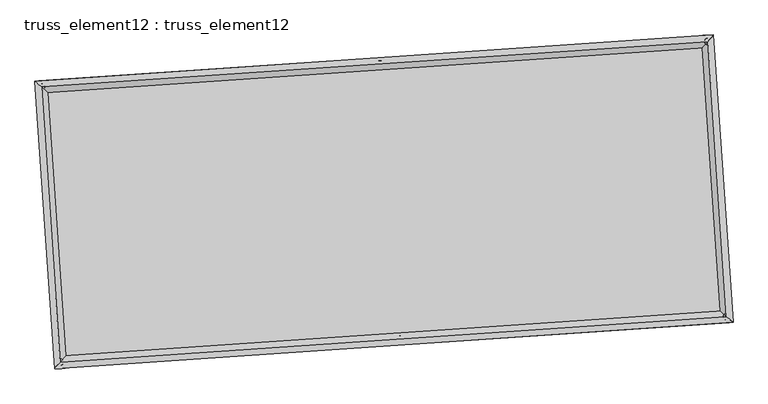
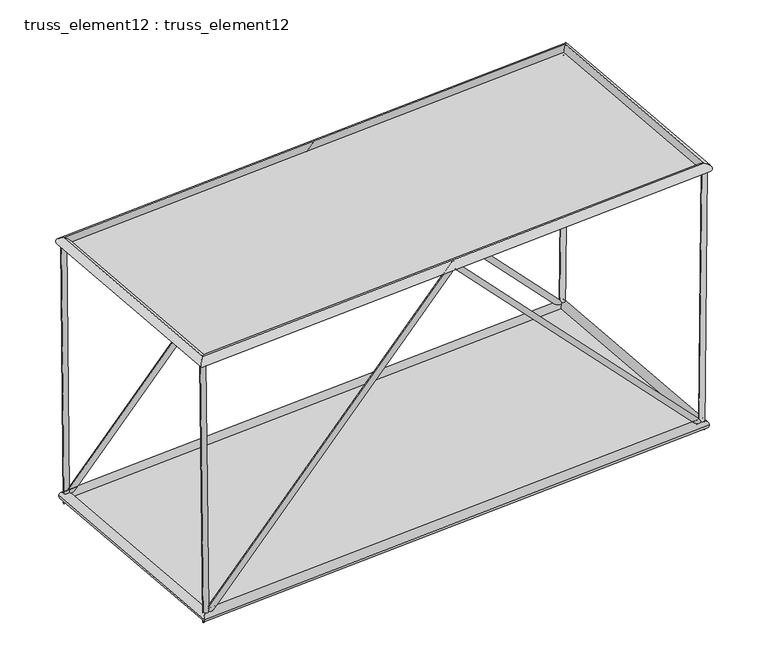
"""IFC4 building model written with IfcOpenShell, lengths in millimetres: plate geometry, truss_element12 : truss_element12."""

from ifc_helpers import new_model, si_unit, frame, origin, origin_with_axes, place, context, project, spatial, polyline, circle_curve, ellipse_curve, outline, extrude, source, transform, mapped, element, save
from ifc_brep_helpers import plane_surface, cylinder_surface, advanced_brep


def truss_element12_truss_element12_25fafcbe(model_context):
    return source(origin(), model_context, "Body", "SolidModel", [
        advanced_brep(
        [(-3717.9336518, 2272.6106472, 5000.2478695), (-3817.0314009, 2259.2497843, 4999.187935), (-3666.2408019, 2276.1353862, 122.8345798), (-3762.7460809, 2262.9512939, -122.8345798), (1064.197845, 2598.6860154, 5071.8345971), (1064.6389029, 2592.1123254, 4927.5910047), (5793.7028088, 2921.1729804, 122.8278987), (5891.0581682, 2921.2075081, -122.8278987), (5846.3222996, 2924.7609034, 5000.2471651), (5946.316249, 2924.9753466, 4999.1682339)],
        [
            (0, 1, circle_curve(frame((-3767.4825264, 2265.9302158, 4999.7179023), z_axis=(-0.01059781698674716, -0.0007226248542523914, 0.9999435804526352), x_axis=(-0.13360875038090175, 0.9910339106331651, -0.0006998548346273042)), 50.0)),
            (1, 0, circle_curve(frame((-3767.4825264, 2265.9302158, 4999.7179023), z_axis=(-0.01059781698674716, -0.0007226248542523914, 0.9999435804526352), x_axis=(-0.13360875038090175, 0.9910339106331651, -0.0006998548346273042)), 50.0)),
            (0, 2),
            (2, 3, ellipse_curve(frame((-3714.4934414, 2269.54334, 0.0), z_axis=(-0.9277371610449594, -0.06325887035254743, 0.36783430418866414), x_axis=(0.36698217779578546, 0.025023119674036753, 0.9298913509986214)), 132.383262, 50.0)),
            (3, 1),
            (3, 2, ellipse_curve(frame((-3714.4934414, 2269.54334, 0.0), z_axis=(-0.9277371610449594, -0.06325887035254743, 0.36783430418866414), x_axis=(0.36698217779578546, 0.025023119674036753, 0.9298913509986214)), 132.383262, 50.0)),
            (2, 4),
            (4, 5, ellipse_curve(frame((1064.418374, 2595.3991704, 4999.7128009), z_axis=(-0.9976833948456157, -0.0680282381448872, 4.9641008010384885e-05), x_axis=(-4.952600945652472e-05, -3.3769903190067476e-06, -0.9999999987678853)), 72.2788404, 50.0)),
            (5, 3),
            (5, 4, ellipse_curve(frame((1064.418374, 2595.3991704, 4999.7128009), z_axis=(-0.9976833948456157, -0.0680282381448872, 4.9641008010384885e-05), x_axis=(-4.952600945652472e-05, -3.3769903190067476e-06, -0.9999999987678853)), 72.2788404, 50.0)),
            (4, 6),
            (6, 7, ellipse_curve(frame((5842.3804885, 2921.1902443, 0.0), z_axis=(-0.9277903039426281, -0.06326249396472418, -0.36769961757854613), x_axis=(-0.3668478032011972, -0.025013957181237265, 0.9299446172931972)), 132.3684791, 50.0)),
            (7, 5),
            (7, 6, ellipse_curve(frame((5842.3804885, 2921.1902443, 0.0), z_axis=(-0.9277903039426281, -0.06326249396472418, -0.36769961757854613), x_axis=(-0.3668478032011972, -0.025013957181237265, 0.9299446172931972)), 132.3684791, 50.0)),
            (8, 9, circle_curve(frame((5896.3192743, 2924.868125, 4999.7076995), z_axis=(0.010787757166797024, 0.0007355761530998497, 0.9999415399027252), x_axis=(-0.0021522428826436795, 0.9999974301665041, -0.0007123980360681724)), 50.0)),
            (9, 8, circle_curve(frame((5896.3192743, 2924.868125, 4999.7076995), z_axis=(0.010787757166797024, 0.0007355761530998497, 0.9999415399027252), x_axis=(-0.0021522428826436795, 0.9999974301665041, -0.0007123980360681724)), 50.0)),
            (6, 8),
            (9, 7),
        ],
        [
            plane_surface(frame((-3767.4825264, 2315.9302027, 4999.7540355), z_axis=(-0.010597816986746694, -0.0007226248542495527, 0.9999435804526353), x_axis=(0.9999438415606726, -7.658676055122278e-06, 0.010597814219416088))),
            cylinder_surface(frame((-3767.4825264, 2265.9302158, 4999.7179023), z_axis=(-0.01059781698674716, -0.0007226248542523914, 0.9999435804526352), x_axis=(-0.13360875038090175, 0.9910339106331651, -0.0006998548346273042)), 50.0),
            cylinder_surface(frame((-3714.4934414, 2269.54334, 0.0), z_axis=(-0.6901986031859024, -0.04706201906073101, -0.7220879825354779), x_axis=(-0.020416121080295117, 0.9987520857397071, -0.045579087645757826)), 50.0),
            cylinder_surface(frame((1064.418374, 2595.3991704, 4999.7128009), z_axis=(-0.690127075511872, -0.04705714186054079, 0.7221566623976738), x_axis=(-0.11534925252048381, 0.9922789563814176, -0.04557436412689142)), 50.0),
            plane_surface(frame((5896.3192743, 2874.8681385, 4999.7444805), z_axis=(0.010787757166796641, 0.0007355761530995457, 0.9999415399027253), x_axis=(0.9999418104546436, -7.935678690174086e-06, -0.010787754247978398))),
            cylinder_surface(frame((5842.3804885, 2921.1902443, 0.0), z_axis=(-0.010787757166797024, -0.0007355761530998497, -0.9999415399027252), x_axis=(-0.0021522428826436795, 0.9999974301665041, -0.0007123980360681724)), 50.0),
        ],
        [
            (0, [[1, 2]]),
            (1, [[-1, 3, 4, 5]]),
            (1, [[-2, -5, 6, -3]]),
            (2, [[-4, 7, 8, 9]]),
            (2, [[-6, -9, 10, -7]]),
            (3, [[-8, 11, 12, 13]]),
            (3, [[-10, -13, 14, -11]]),
            (4, [[15, 16]]),
            (5, [[-12, 17, -16, 18]]),
            (5, [[-14, -18, -15, -17]]),
        ],
    ),
        advanced_brep(
        [(-3445.8206989, -1718.1229371, 5000.2478695), (-3544.918448, -1731.4838, 4999.187935), (-3394.127849, -1714.5981981, 122.8345798), (-3490.633128, -1727.7822904, -122.8345798), (1336.310798, -1392.0475689, 5071.8345971), (1336.7518559, -1398.6212589, 4927.5910047), (6065.8157618, -1069.5606039, 122.8278987), (6163.1711211, -1069.5260762, -122.8278987), (6118.4352525, -1065.9726809, 5000.2471651), (6218.429202, -1065.7582377, 4999.1682339)],
        [
            (0, 1, circle_curve(frame((-3495.3695734, -1724.8033685, 4999.7179023), z_axis=(-0.01059781698674734, -0.0007226248542523697, 0.9999435804526352), x_axis=(-0.13360875038090145, 0.9910339106331651, -0.000699854834627346)), 50.0)),
            (1, 0, circle_curve(frame((-3495.3695734, -1724.8033685, 4999.7179023), z_axis=(-0.01059781698674734, -0.0007226248542523697, 0.9999435804526352), x_axis=(-0.13360875038090145, 0.9910339106331651, -0.000699854834627346)), 50.0)),
            (0, 2),
            (2, 3, ellipse_curve(frame((-3442.3804885, -1721.1902443, 0.0), z_axis=(-0.9277371610449594, -0.06325887035254724, 0.3678343041886641), x_axis=(0.3669821777957854, 0.02502311967403671, 0.9298913509986214)), 132.383262, 50.0)),
            (3, 1),
            (3, 2, ellipse_curve(frame((-3442.3804885, -1721.1902443, 0.0), z_axis=(-0.9277371610449594, -0.06325887035254724, 0.3678343041886641), x_axis=(0.3669821777957854, 0.02502311967403671, 0.9298913509986214)), 132.383262, 50.0)),
            (2, 4),
            (4, 5, ellipse_curve(frame((1336.5313269, -1395.3344139, 4999.7128009), z_axis=(-0.9976833948456157, -0.06802823814488712, 4.964100801046513e-05), x_axis=(-4.952600945652472e-05, -3.3769903189394843e-06, -0.9999999987678853)), 72.2788404, 50.0)),
            (5, 3),
            (5, 4, ellipse_curve(frame((1336.5313269, -1395.3344139, 4999.7128009), z_axis=(-0.9976833948456157, -0.06802823814488712, 4.964100801046513e-05), x_axis=(-4.952600945652472e-05, -3.3769903189394843e-06, -0.9999999987678853)), 72.2788404, 50.0)),
            (4, 6),
            (6, 7, ellipse_curve(frame((6114.4934414, -1069.54334, 0.0), z_axis=(-0.9277903039426281, -0.06326249396472412, -0.3676996175785463), x_axis=(-0.36684780320119736, -0.025013957181237296, 0.9299446172931972)), 132.3684791, 50.0)),
            (7, 5),
            (7, 6, ellipse_curve(frame((6114.4934414, -1069.54334, 0.0), z_axis=(-0.9277903039426281, -0.06326249396472412, -0.3676996175785463), x_axis=(-0.36684780320119736, -0.025013957181237296, 0.9299446172931972)), 132.3684791, 50.0)),
            (8, 9, circle_curve(frame((6168.4322273, -1065.8654593, 4999.7076995), z_axis=(0.010787757166797012, 0.00073557615309981, 0.9999415399027253), x_axis=(-0.0021522428826438933, 0.9999974301665041, -0.0007123980360681303)), 50.0)),
            (9, 8, circle_curve(frame((6168.4322273, -1065.8654593, 4999.7076995), z_axis=(0.010787757166797012, 0.00073557615309981, 0.9999415399027253), x_axis=(-0.0021522428826438933, 0.9999974301665041, -0.0007123980360681303)), 50.0)),
            (6, 8),
            (9, 7),
        ],
        [
            plane_surface(frame((-3495.3695734, -1674.8033816, 4999.7540355), z_axis=(-0.010597816986746694, -0.0007226248542495488, 0.9999435804526353), x_axis=(0.9999438415606726, -7.658676055122278e-06, 0.010597814219416088))),
            cylinder_surface(frame((-3495.3695734, -1724.8033685, 4999.7179023), z_axis=(-0.01059781698674734, -0.0007226248542523697, 0.9999435804526352), x_axis=(-0.13360875038090145, 0.9910339106331651, -0.000699854834627346)), 50.0),
            cylinder_surface(frame((-3442.3804885, -1721.1902443, 0.0), z_axis=(-0.6901986031859025, -0.0470620190607309, -0.7220879825354778), x_axis=(-0.0204161210802951, 0.9987520857397071, -0.0455790876457577)), 50.0),
            cylinder_surface(frame((1336.5313269, -1395.3344139, 4999.7128009), z_axis=(-0.6901270755118721, -0.047057141860540795, 0.722156662397674), x_axis=(-0.11534925252048368, 0.9922789563814176, -0.0455743641268913)), 50.0),
            plane_surface(frame((6168.4322273, -1115.8654458, 4999.7444805), z_axis=(0.010787757166796641, 0.0007355761530995437, 0.9999415399027253), x_axis=(0.9999418104546436, -7.935678691062265e-06, -0.010787754247978398))),
            cylinder_surface(frame((6114.4934414, -1069.54334, 0.0), z_axis=(-0.010787757166797012, -0.00073557615309981, -0.9999415399027253), x_axis=(-0.0021522428826438933, 0.9999974301665041, -0.0007123980360681303)), 50.0),
        ],
        [
            (0, [[1, 2]]),
            (1, [[-1, 3, 4, 5]]),
            (1, [[-2, -5, 6, -3]]),
            (2, [[-4, 7, 8, 9]]),
            (2, [[-6, -9, 10, -7]]),
            (3, [[-8, 11, 12, 13]]),
            (3, [[-10, -13, 14, -11]]),
            (4, [[15, 16]]),
            (5, [[-12, 17, -16, 18]]),
            (5, [[-14, -18, -15, -17]]),
        ],
    ),
        advanced_brep(
        [(-3495.372256, -1724.8063417, 4909.7179023), (-3495.3668909, -1724.8003953, 5089.7179022), (-3767.479465, 2265.9276342, 5089.7179022), (-3767.4855877, 2265.9327973, 4909.7179023), (5896.3167809, 2924.8651647, 5089.7076995), (5896.3217678, 2924.8710853, 4909.7076996), (6168.4293551, -1065.8628648, 5089.7076995), (6168.4350994, -1065.8680537, 4909.7076996)],
        [
            (0, 1, ellipse_curve(frame((-3495.3695734, -1724.8033685, 4999.7179023), z_axis=(-0.7535719234050675, 0.6573654662781063, 7.448125025781954e-07), x_axis=(-0.6573654662776883, -0.7535719234054323, 7.448125025782821e-07)), 127.2792206, 90.0)),
            (1, 2),
            (2, 3, ellipse_curve(frame((-3767.4825264, 2265.9302158, 4999.7179023), z_axis=(-0.6573654662776883, -0.7535719234054322, 7.448125025783611e-07), x_axis=(0.7535719234050674, -0.6573654662781064, -7.44812502578274e-07)), 127.2792206, 90.0)),
            (3, 0),
            (1, 0, ellipse_curve(frame((-3495.3695734, -1724.8033685, 4999.7179023), z_axis=(-0.7535719234050675, 0.6573654662781063, 7.448125025781954e-07), x_axis=(-0.6573654662776883, -0.7535719234054323, 7.448125025782821e-07)), 127.2792206, 90.0)),
            (3, 2, ellipse_curve(frame((-3767.4825264, 2265.9302158, 4999.7179023), z_axis=(-0.6573654662776883, -0.7535719234054322, 7.448125025783611e-07), x_axis=(0.7535719234050674, -0.6573654662781064, -7.44812502578274e-07)), 127.2792206, 90.0)),
            (2, 4),
            (4, 5, ellipse_curve(frame((5896.3192743, 2924.868125, 4999.7076995), z_axis=(-0.7535719234050677, 0.6573654662781063, 7.448125025783542e-07), x_axis=(-0.6573654662776882, -0.7535719234054323, 7.448125025782813e-07)), 127.2792206, 90.0)),
            (5, 3),
            (5, 4, ellipse_curve(frame((5896.3192743, 2924.868125, 4999.7076995), z_axis=(-0.7535719234050677, 0.6573654662781063, 7.448125025783542e-07), x_axis=(-0.6573654662776882, -0.7535719234054323, 7.448125025782813e-07)), 127.2792206, 90.0)),
            (4, 6),
            (6, 7, ellipse_curve(frame((6168.4322273, -1065.8654593, 4999.7076995), z_axis=(0.6573654662776882, 0.7535719234054323, -7.448125025782022e-07), x_axis=(-0.7535719234050676, 0.6573654662781062, 7.448125025782751e-07)), 127.2792206, 90.0)),
            (7, 5),
            (7, 6, ellipse_curve(frame((6168.4322273, -1065.8654593, 4999.7076995), z_axis=(0.6573654662776882, 0.7535719234054323, -7.448125025782022e-07), x_axis=(-0.7535719234050676, 0.6573654662781062, 7.448125025782751e-07)), 127.2792206, 90.0)),
            (6, 1),
            (0, 7),
        ],
        [
            cylinder_surface(frame((-3495.3695734, -1724.8033685, 4999.7179023), z_axis=(0.06802823822870346, -0.9976833960748764, 0.0), x_axis=(-0.9976833955645505, -0.06802823819390627, 3.1984710746243846e-05)), 90.0),
            cylinder_surface(frame((-3767.4825264, 2265.9302158, 4999.7179023), z_axis=(-0.9976833960743232, -0.06802823822866429, 1.053323942571303e-06), x_axis=(-0.0680282381636537, 0.9976833955998259, 3.093138680417647e-05)), 90.0),
            cylinder_surface(frame((5896.3192743, 2924.868125, 4999.7076995), z_axis=(-0.06802823822870388, 0.9976833960748765, 0.0), x_axis=(0.9976833956295612, 0.06802823819833952, 2.9878062862109108e-05)), 90.0),
            cylinder_surface(frame((6168.4322273, -1065.8654593, 4999.7076995), z_axis=(0.9976833960743232, 0.06802823822866422, -1.0533239425711911e-06), x_axis=(0.06802823822866422, -0.9976833955953931, 3.093138680417647e-05)), 90.0),
        ],
        [
            (0, [[1, 2, 3, 4]]),
            (0, [[5, -4, 6, -2]]),
            (1, [[-3, 7, 8, 9]]),
            (1, [[-6, -9, 10, -7]]),
            (2, [[-8, 11, 12, 13]]),
            (2, [[-10, -13, 14, -11]]),
            (3, [[-12, 15, -1, 16]]),
            (3, [[-14, -16, -5, -15]]),
        ],
    ),
        advanced_brep(
        [(-3358.7115243, -1625.2761972, 0.0), (-3526.0494527, -1817.1042913, 0.0), (-3810.4074885, 2353.2123043, 0.0), (-3618.5793943, 2185.8743758, 0.0), (5926.0494527, 3017.1042913, 0.0), (5758.7115243, 2825.2761972, 0.0), (6210.4074885, -1153.2123043, 0.0), (6018.5793943, -985.8743758, 0.0)],
        [
            (0, 1, ellipse_curve(frame((-3442.3804885, -1721.1902443, 0.0), z_axis=(-0.7535719234054613, 0.6573654662780769, 0.0), x_axis=(-0.6573654662780767, -0.7535719234054614, 0.0)), 127.2792206, 90.0)),
            (1, 2),
            (2, 3, ellipse_curve(frame((-3714.4934414, 2269.54334, 0.0), z_axis=(-0.6573654662780768, -0.7535719234054614, 0.0), x_axis=(0.7535719234054613, -0.6573654662780768, 0.0)), 127.2792206, 90.0)),
            (3, 0),
            (1, 0, ellipse_curve(frame((-3442.3804885, -1721.1902443, 0.0), z_axis=(-0.7535719234054613, 0.6573654662780769, 0.0), x_axis=(-0.6573654662780767, -0.7535719234054614, 0.0)), 127.2792206, 90.0)),
            (3, 2, ellipse_curve(frame((-3714.4934414, 2269.54334, 0.0), z_axis=(-0.6573654662780768, -0.7535719234054614, 0.0), x_axis=(0.7535719234054613, -0.6573654662780768, 0.0)), 127.2792206, 90.0)),
            (2, 4),
            (4, 5, ellipse_curve(frame((5842.3804885, 2921.1902443, 0.0), z_axis=(-0.7535719234054613, 0.6573654662780768, 0.0), x_axis=(-0.657365466278077, -0.7535719234054612, 0.0)), 127.2792206, 90.0)),
            (5, 3),
            (5, 4, ellipse_curve(frame((5842.3804885, 2921.1902443, 0.0), z_axis=(-0.7535719234054613, 0.6573654662780768, 0.0), x_axis=(-0.657365466278077, -0.7535719234054612, 0.0)), 127.2792206, 90.0)),
            (4, 6),
            (6, 7, ellipse_curve(frame((6114.4934414, -1069.54334, 0.0), z_axis=(0.657365466278077, 0.7535719234054614, 0.0), x_axis=(-0.7535719234054615, 0.6573654662780768, 0.0)), 127.2792206, 90.0)),
            (7, 5),
            (7, 6, ellipse_curve(frame((6114.4934414, -1069.54334, 0.0), z_axis=(0.657365466278077, 0.7535719234054614, 0.0), x_axis=(-0.7535719234054615, 0.6573654662780768, 0.0)), 127.2792206, 90.0)),
            (6, 1),
            (0, 7),
        ],
        [
            cylinder_surface(frame((-3442.3804885, -1721.1902443, 0.0), z_axis=(0.06802823822870728, -0.9976833960748762, 0.0), x_axis=(-0.9976833960748762, -0.06802823822870728, 0.0)), 90.0),
            cylinder_surface(frame((-3714.4934414, 2269.54334, 0.0), z_axis=(-0.9976833960748763, -0.06802823822870568, 0.0), x_axis=(-0.06802823822870568, 0.9976833960748763, 0.0)), 90.0),
            cylinder_surface(frame((5842.3804885, 2921.1902443, 0.0), z_axis=(-0.0680282382287072, 0.9976833960748762, 0.0), x_axis=(0.9976833960748762, 0.0680282382287072, 0.0)), 90.0),
            cylinder_surface(frame((6114.4934414, -1069.54334, 0.0), z_axis=(0.9976833960748763, 0.0680282382287056, 0.0), x_axis=(0.0680282382287056, -0.9976833960748763, 0.0)), 90.0),
        ],
        [
            (0, [[1, 2, 3, 4]]),
            (0, [[5, -4, 6, -2]]),
            (1, [[-3, 7, 8, 9]]),
            (1, [[-6, -9, 10, -7]]),
            (2, [[-8, 11, 12, 13]]),
            (2, [[-10, -13, 14, -11]]),
            (3, [[-12, 15, -1, 16]]),
            (3, [[-14, -16, -5, -15]]),
        ],
    ),
        extrude(outline(polyline([(-3442.3804885, -1721.1902443), (-3714.4934414, 2269.54334), (5842.3804885, 2921.1902443), (6114.4934414, -1069.54334), (-3442.3804885, -1721.1902443)])), origin_with_axes(), (0.0, 0.0, 1.0), 20.0),
        extrude(outline(polyline([(-1999.9999999, 4843.1204923), (2000.0000001, 4843.1204924), (2000.0, -4843.1204922), (-2000.0, -4843.1204923), (-1999.9999999, 4843.1204923)])), frame((1200.4748505, 600.0323782, 4999.7128009), z_axis=(1.0508838081914596e-06, 7.165577209723778e-08, 0.9999999999994453), x_axis=(-0.06802823822870709, 0.9976833960748762, 0.0)), (0.0, 0.0, 1.0), 20.0),
    ])


if __name__ == "__main__":
    model = new_model("IFC4")
    model_context = context("Model", 3, world=origin())
    ifc_project = project(units=[si_unit("LENGTHUNIT", "METRE", prefix="MILLI")], contexts=[model_context])
    site = spatial("IfcSite", under=ifc_project)
    building = spatial("IfcBuilding", under=site)
    placement = place(None, origin())
    truss_element12_truss_element12_shape = truss_element12_truss_element12_25fafcbe(model_context)
    element("IfcPlate", 1, ObjectType="truss_element12 : truss_element12", at=placement, inside=building, context=model_context, shape_type="MappedRepresentation", body=[
        mapped(truss_element12_truss_element12_shape, transform((0.0, 0.0, 0.0), x_axis=(1.0, 0.0, 0.0), y_axis=(0.0, 1.0, 0.0), z_axis=(0.0, 0.0, 1.0))),
    ])
    save(model, "model.ifc")

# Revit data of these elements
# Type "truss_element12 : truss_element12"
#   steellbar1 = 90 mm
#   steelbar2 = 50 mm
#   offset1 = 5000 mm
#   M = Default Roof
# Element 1 (IfcPlate, "truss_element12 : truss_element12")
#   Materials on its faces: "Default Roof"
# Materials
#   "Default Roof": class "Miscellaneous", colour RGB 0 127 0, transparency 0, Comments = "Rendering appearance not upgraded Rendering appearance not upgraded ", Cost = 0
